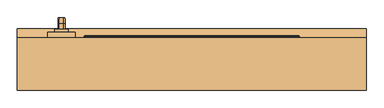
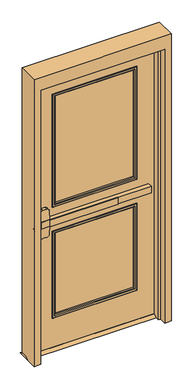
"""IFC4 building model written with IfcOpenShell, lengths in millimetres: door geometry, Дверь-Наружная-Одинарная-Две_Свет : Дверь-Наружная-Одинарная-Две_Свет."""

from ifc_helpers import new_model, si_unit, point, frame, frame_2d, origin, place, context, project, spatial, polyline, circle_curve, ellipse_curve, trimmed, segment, composite_curve, outline, extrude, faceted_brep, source, transform, mapped, element, save
from ifc_brep_helpers import plane_surface, cylinder_surface, revolved_surface, advanced_brep


def door_4063ef7d(model_context):
    return source(origin(), model_context, "Body", "SolidModel", [
        extrude(outline(polyline([(36.35, 15.0), (81.35, 15.0), (106.75, 0.0), (10.95, 0.0), (36.35, 15.0)])), frame((-500.0, 0.0, 0.0), z_axis=(1.0, 0.0, 0.0), x_axis=(0.0, 1.0, 0.0)), (0.0, 0.0, 1.0), 1000.0),
        extrude(outline(polyline([(148.95, -1.75), (-342.05, -1.75), (-342.05, 4.6), (148.95, 4.6), (148.95, -1.75)])), frame((0.0, 0.0, 974.6), z_axis=(0.0, 0.0, 1.0), x_axis=(1.0, 0.0, 0.0)), (0.0, 0.0, 1.0), 50.8),
        advanced_brep(
        [(-405.55, 4.6, 1025.4), (-405.55, 4.6, 974.6), (-342.05, 4.6, 974.6), (394.45, 4.6, 974.6), (394.45, 4.6, 1025.4), (-342.05, 4.6, 1025.4), (394.45, 36.35, 1025.4), (394.45, 36.35, 974.6), (-342.05, 36.35, 974.6), (-342.05, 36.35, 911.1), (-361.1, 36.35, 892.05), (-386.5, 36.35, 892.05), (-405.55, 36.35, 911.1), (-405.55, 36.35, 1088.9), (-386.5, 36.35, 1107.95), (-361.1, 36.35, 1107.95), (-342.05, 36.35, 1088.9), (-342.05, 36.35, 1025.4), (-342.05, 7.7752467, 1025.4), (-405.55, 7.7752467, 1025.4), (-405.55, 12.7854269, 1088.9), (-405.55, 12.7854269, 911.1), (-405.55, 7.7752467, 974.6), (-342.05, 7.7752467, 974.6), (-342.05, 12.7854269, 911.1), (-342.05, 12.7854269, 1088.9), (-386.5, 14.288481, 1107.95), (-361.1, 14.288481, 1107.95), (-361.1, 14.288481, 892.05), (-386.5, 14.288481, 892.05)],
        [
            (0, 1),
            (1, 2),
            (2, 3),
            (3, 4),
            (4, 5),
            (5, 0),
            (6, 7),
            (7, 8),
            (8, 9),
            (9, 10, circle_curve(frame((-361.1, 36.35, 911.1), z_axis=(0.0, 1.0, 0.0), x_axis=(1.0, 0.0, 0.0)), 19.05)),
            (10, 11),
            (11, 12, circle_curve(frame((-386.5, 36.35, 911.1), z_axis=(0.0, 1.0, 0.0), x_axis=(1.0, 0.0, 0.0)), 19.05)),
            (12, 13),
            (13, 14, circle_curve(frame((-386.5, 36.35, 1088.9), z_axis=(0.0, 1.0, 0.0), x_axis=(1.0, 0.0, 0.0)), 19.05)),
            (14, 15),
            (15, 16, circle_curve(frame((-361.1, 36.35, 1088.9), z_axis=(0.0, 1.0, 0.0), x_axis=(1.0, 0.0, 0.0)), 19.05)),
            (16, 17),
            (17, 6),
            (4, 6),
            (17, 18),
            (18, 19),
            (19, 0),
            (19, 20),
            (20, 13),
            (12, 21),
            (21, 22),
            (22, 1),
            (7, 3),
            (22, 23),
            (23, 8),
            (23, 24),
            (24, 9),
            (16, 25),
            (25, 18),
            (14, 26),
            (26, 27),
            (27, 15),
            (10, 28),
            (28, 29),
            (29, 11),
            (24, 28, ellipse_curve(frame((-361.1, 12.7854269, 911.1), z_axis=(0.0, 0.9969018152893365, 0.07865602756830282), x_axis=(0.0, -0.07865602756830208, 0.9969018152893365)), 19.1092038, 19.05)),
            (27, 25, ellipse_curve(frame((-361.1, 12.7854269, 1088.9), z_axis=(0.0, 0.9969018152893376, -0.07865602756828934), x_axis=(0.0, -0.078656027568288, -0.9969018152893377)), 19.1092038, 19.05)),
            (20, 26, ellipse_curve(frame((-386.5, 12.7854269, 1088.9), z_axis=(0.0, 0.9969018152893376, -0.07865602756828934), x_axis=(0.0, -0.078656027568288, -0.9969018152893377)), 19.1092038, 19.05)),
            (29, 21, ellipse_curve(frame((-386.5, 12.7854269, 911.1), z_axis=(0.0, 0.9969018152893365, 0.07865602756830282), x_axis=(0.0, -0.07865602756830208, 0.9969018152893365)), 19.1092038, 19.05)),
        ],
        [
            plane_surface(frame((-405.55, 4.6, 1025.4), z_axis=(0.0, -1.0, 0.0), x_axis=(-1.0, 0.0, 0.0))),
            plane_surface(frame((-405.55, 36.35, 1025.4), z_axis=(0.0, 1.0, 0.0), x_axis=(1.0, 0.0, 0.0))),
            plane_surface(frame((394.45, 4.6, 1025.4), z_axis=(0.0, 0.0, 1.0), x_axis=(0.0, 1.0, 0.0))),
            plane_surface(frame((-405.55, 4.6, 1025.4), z_axis=(-1.0, 0.0, 0.0), x_axis=(0.0, 1.0, 0.0))),
            plane_surface(frame((-405.55, 4.6, 974.6), z_axis=(0.0, 0.0, -1.0), x_axis=(0.0, 1.0, 0.0))),
            plane_surface(frame((394.45, 4.6, 974.6), z_axis=(1.0, 0.0, 0.0), x_axis=(0.0, 1.0, 0.0))),
            plane_surface(frame((-342.05, 7.7752467, 911.1), z_axis=(1.0, 0.0, 0.0), x_axis=(0.0, 1.0, 0.0))),
            plane_surface(frame((-361.1, 7.7752467, 1107.95), z_axis=(0.0, 0.0, 1.0), x_axis=(0.0, 1.0, 0.0))),
            plane_surface(frame((-386.5, 7.7752467, 892.05), z_axis=(0.0, 0.0, -1.0), x_axis=(0.0, 1.0, 0.0))),
            cylinder_surface(frame((-361.1, 36.35, 911.1), z_axis=(0.0, -1.0, 0.0), x_axis=(1.0, 0.0, 0.0)), 19.05),
            cylinder_surface(frame((-361.1, 36.35, 1088.9), z_axis=(0.0, -1.0, 0.0), x_axis=(1.0, 0.0, 0.0)), 19.05),
            cylinder_surface(frame((-386.5, 36.35, 1088.9), z_axis=(0.0, -1.0, 0.0), x_axis=(1.0, 0.0, 0.0)), 19.05),
            cylinder_surface(frame((-386.5, 36.35, 911.1), z_axis=(0.0, -1.0, 0.0), x_axis=(1.0, 0.0, 0.0)), 19.05),
            plane_surface(frame((-342.05, 7.7752467, 1025.4), z_axis=(0.0, -0.9969018152893376, 0.07865602756828934), x_axis=(-1.0, 0.0, 0.0))),
            plane_surface(frame((-342.05, 14.288481, 892.05), z_axis=(0.0, -0.9969018152893365, -0.07865602756830282), x_axis=(-1.0, 0.0, 0.0))),
        ],
        [
            (0, [[1, 2, 3, 4, 5, 6]]),
            (1, [[7, 8, 9, 10, 11, 12, 13, 14, 15, 16, 17, 18]]),
            (2, [[19, -18, 20, 21, 22, -6, -5]]),
            (3, [[-1, -22, 23, 24, -13, 25, 26, 27]]),
            (4, [[28, -3, -2, -27, 29, 30, -8]]),
            (5, [[-4, -28, -7, -19]]),
            (6, [[-9, -30, 31, 32]]),
            (6, [[-17, 33, 34, -20]]),
            (7, [[-15, 35, 36, 37]]),
            (8, [[-11, 38, 39, 40]]),
            (9, [[-10, -32, 41, -38]]),
            (10, [[-16, -37, 42, -33]]),
            (11, [[-14, -24, 43, -35]]),
            (12, [[-12, -40, 44, -25]]),
            (13, [[-21, -34, -42, -36, -43, -23]]),
            (14, [[-26, -44, -39, -41, -31, -29]]),
        ],
    ),
        advanced_brep(
        [(-383.8, 96.35, 1001.190625), (-383.8, 96.35, 998.809375), (-380.228125, 96.35, 995.2375), (-367.3715406, 96.35, 995.2375), (-363.8, 96.35, 998.8090406), (-363.8, 96.35, 1001.190625), (-367.371875, 96.35, 1004.7625), (-380.228125, 96.35, 1004.7625), (-383.8, 96.35, 874.609375), (-380.228125, 96.35, 871.0375), (-367.371875, 96.35, 871.0375), (-363.8, 96.35, 874.609375), (-363.8, 96.35, 876.9909594), (-367.3715406, 96.35, 880.5625), (-380.228125, 96.35, 880.5625), (-383.8, 96.35, 876.990625), (-383.8, 121.75, 1001.190625), (-383.8, 135.640625, 987.3), (-383.8, 135.640625, 888.5), (-383.8, 121.75, 874.609375), (-383.8, 121.75, 876.990625), (-383.8, 133.259375, 888.5), (-383.8, 133.259375, 987.3), (-383.8, 121.75, 998.809375), (-380.228125, 121.75, 995.2375), (-367.3715406, 121.75, 995.2375), (-363.8, 121.75, 998.8090406), (-363.8, 133.2590406, 987.3), (-363.8, 133.2590406, 888.5), (-363.8, 121.75, 876.9909594), (-363.8, 121.75, 874.609375), (-363.8, 135.640625, 888.5), (-363.8, 135.640625, 987.3), (-363.8, 121.75, 1001.190625), (-367.371875, 121.75, 1004.7625), (-380.228125, 121.75, 1004.7625), (-380.228125, 129.6875, 987.3), (-367.3715406, 129.6875, 987.3), (-367.371875, 139.2125, 987.3), (-380.228125, 139.2125, 987.3), (-380.228125, 129.6875, 888.5), (-367.3715406, 129.6875, 888.5), (-367.371875, 139.2125, 888.5), (-380.228125, 139.2125, 888.5), (-380.228125, 121.75, 880.5625), (-367.3715406, 121.75, 880.5625), (-367.371875, 121.75, 871.0375), (-380.228125, 121.75, 871.0375)],
        [
            (0, 1),
            (1, 2, circle_curve(frame((-380.228125, 96.35, 998.809375), z_axis=(0.0, -1.0, 0.0), x_axis=(0.0, 0.0, 1.0)), 3.571875)),
            (2, 3),
            (3, 4, circle_curve(frame((-367.3715406, 96.35, 998.8090406), z_axis=(0.0, -1.0, 0.0), x_axis=(0.0, 0.0, 1.0)), 3.5715406)),
            (4, 5),
            (5, 6, circle_curve(frame((-367.371875, 96.35, 1001.190625), z_axis=(0.0, -1.0, 0.0), x_axis=(0.0, 0.0, 1.0)), 3.571875)),
            (6, 7),
            (7, 0, circle_curve(frame((-380.228125, 96.35, 1001.190625), z_axis=(0.0, -1.0, 0.0), x_axis=(0.0, 0.0, 1.0)), 3.571875)),
            (8, 9, circle_curve(frame((-380.228125, 96.35, 874.609375), z_axis=(0.0, -1.0, 0.0), x_axis=(0.0, 0.0, -1.0)), 3.571875)),
            (9, 10),
            (10, 11, circle_curve(frame((-367.371875, 96.35, 874.609375), z_axis=(0.0, -1.0, 0.0), x_axis=(0.0, 0.0, -1.0)), 3.571875)),
            (11, 12),
            (12, 13, circle_curve(frame((-367.3715406, 96.35, 876.9909594), z_axis=(0.0, -1.0, 0.0), x_axis=(0.0, 0.0, -1.0)), 3.5715406)),
            (13, 14),
            (14, 15, circle_curve(frame((-380.228125, 96.35, 876.990625), z_axis=(0.0, -1.0, 0.0), x_axis=(0.0, 0.0, -1.0)), 3.571875)),
            (15, 8),
            (0, 16),
            (16, 17, circle_curve(frame((-383.8, 121.75, 987.3), z_axis=(-1.0, 0.0, 0.0), x_axis=(0.0, 0.0, 1.0)), 13.890625)),
            (17, 18),
            (18, 19, circle_curve(frame((-383.8, 121.75, 888.5), z_axis=(-1.0, 0.0, 0.0), x_axis=(0.0, 1.0, 0.0)), 13.890625)),
            (19, 8),
            (15, 20),
            (20, 21, circle_curve(frame((-383.8, 121.75, 888.5), z_axis=(1.0, 0.0, 0.0), x_axis=(0.0, 1.0, 0.0)), 11.509375)),
            (21, 22),
            (22, 23, circle_curve(frame((-383.8, 121.75, 987.3), z_axis=(1.0, 0.0, 0.0), x_axis=(0.0, 0.0, 1.0)), 11.509375)),
            (23, 1),
            (23, 24, circle_curve(frame((-380.228125, 121.75, 998.809375), z_axis=(0.0, -1.0, 0.0), x_axis=(0.0, 0.0, 1.0)), 3.571875)),
            (24, 2),
            (24, 25),
            (25, 3),
            (25, 26, circle_curve(frame((-367.3715406, 121.75, 998.8090406), z_axis=(0.0, -1.0, 0.0), x_axis=(0.0, 0.0, 1.0)), 3.5715406)),
            (26, 4),
            (26, 27, circle_curve(frame((-363.8, 121.75, 987.3), z_axis=(-1.0, 0.0, 0.0), x_axis=(0.0, 0.0, 1.0)), 11.5090406)),
            (27, 28),
            (28, 29, circle_curve(frame((-363.8, 121.75, 888.5), z_axis=(-1.0, 0.0, 0.0), x_axis=(0.0, 1.0, 0.0)), 11.5090406)),
            (29, 12),
            (11, 30),
            (30, 31, circle_curve(frame((-363.8, 121.75, 888.5), z_axis=(1.0, 0.0, 0.0), x_axis=(0.0, 1.0, 0.0)), 13.890625)),
            (31, 32),
            (32, 33, circle_curve(frame((-363.8, 121.75, 987.3), z_axis=(1.0, 0.0, 0.0), x_axis=(0.0, 0.0, 1.0)), 13.890625)),
            (33, 5),
            (33, 34, circle_curve(frame((-367.371875, 121.75, 1001.190625), z_axis=(0.0, -1.0, 0.0), x_axis=(0.0, 0.0, 1.0)), 3.571875)),
            (34, 6),
            (34, 35),
            (35, 7),
            (35, 16, circle_curve(frame((-380.228125, 121.75, 1001.190625), z_axis=(0.0, -1.0, 0.0), x_axis=(0.0, 0.0, 1.0)), 3.571875)),
            (36, 24, circle_curve(frame((-380.228125, 121.75, 987.3), z_axis=(1.0, 0.0, 0.0), x_axis=(0.0, 0.0, 1.0)), 7.9375)),
            (22, 36, circle_curve(frame((-380.228125, 133.259375, 987.3), z_axis=(0.0, 0.0, 1.0), x_axis=(0.0, 1.0, 0.0)), 3.571875)),
            (37, 25, circle_curve(frame((-367.3715406, 121.75, 987.3), z_axis=(1.0, 0.0, 0.0), x_axis=(0.0, 0.0, 1.0)), 7.9375)),
            (36, 37),
            (37, 27, circle_curve(frame((-367.3715406, 133.2590406, 987.3), z_axis=(0.0, 0.0, 1.0), x_axis=(0.0, 1.0, 0.0)), 3.5715406)),
            (38, 34, circle_curve(frame((-367.371875, 121.75, 987.3), z_axis=(1.0, 0.0, 0.0), x_axis=(0.0, 0.0, 1.0)), 17.4625)),
            (32, 38, circle_curve(frame((-367.371875, 135.640625, 987.3), z_axis=(0.0, 0.0, 1.0), x_axis=(0.0, 1.0, 0.0)), 3.571875)),
            (39, 35, circle_curve(frame((-380.228125, 121.75, 987.3), z_axis=(1.0, 0.0, 0.0), x_axis=(0.0, 0.0, 1.0)), 17.4625)),
            (38, 39),
            (39, 17, circle_curve(frame((-380.228125, 135.640625, 987.3), z_axis=(0.0, 0.0, 1.0), x_axis=(0.0, 1.0, 0.0)), 3.571875)),
            (21, 40, circle_curve(frame((-380.228125, 133.259375, 888.5), z_axis=(0.0, 0.0, 1.0), x_axis=(0.0, 1.0, 0.0)), 3.571875)),
            (40, 36),
            (40, 41),
            (41, 37),
            (41, 28, circle_curve(frame((-367.3715406, 133.2590406, 888.5), z_axis=(0.0, 0.0, 1.0), x_axis=(0.0, 1.0, 0.0)), 3.5715406)),
            (31, 42, circle_curve(frame((-367.371875, 135.640625, 888.5), z_axis=(0.0, 0.0, 1.0), x_axis=(0.0, 1.0, 0.0)), 3.571875)),
            (42, 38),
            (42, 43),
            (43, 39),
            (43, 18, circle_curve(frame((-380.228125, 135.640625, 888.5), z_axis=(0.0, 0.0, 1.0), x_axis=(0.0, 1.0, 0.0)), 3.571875)),
            (44, 40, circle_curve(frame((-380.228125, 121.75, 888.5), z_axis=(1.0, 0.0, 0.0), x_axis=(0.0, 1.0, 0.0)), 7.9375)),
            (20, 44, circle_curve(frame((-380.228125, 121.75, 876.990625), z_axis=(0.0, 1.0, 0.0), x_axis=(0.0, 0.0, -1.0)), 3.571875)),
            (45, 41, circle_curve(frame((-367.3715406, 121.75, 888.5), z_axis=(1.0, 0.0, 0.0), x_axis=(0.0, 1.0, 0.0)), 7.9375)),
            (44, 45),
            (45, 29, circle_curve(frame((-367.3715406, 121.75, 876.9909594), z_axis=(0.0, 1.0, 0.0), x_axis=(0.0, 0.0, -1.0)), 3.5715406)),
            (46, 42, circle_curve(frame((-367.371875, 121.75, 888.5), z_axis=(1.0, 0.0, 0.0), x_axis=(0.0, 1.0, 0.0)), 17.4625)),
            (30, 46, circle_curve(frame((-367.371875, 121.75, 874.609375), z_axis=(0.0, 1.0, 0.0), x_axis=(0.0, 0.0, -1.0)), 3.571875)),
            (47, 43, circle_curve(frame((-380.228125, 121.75, 888.5), z_axis=(1.0, 0.0, 0.0), x_axis=(0.0, 1.0, 0.0)), 17.4625)),
            (46, 47),
            (47, 19, circle_curve(frame((-380.228125, 121.75, 874.609375), z_axis=(0.0, 1.0, 0.0), x_axis=(0.0, 0.0, -1.0)), 3.571875)),
            (14, 44),
            (13, 45),
            (10, 46),
            (9, 47),
        ],
        [
            plane_surface(frame((-373.8, 96.35, 1000.0), z_axis=(0.0, -1.0, 0.0), x_axis=(1.0, 0.0, 0.0))),
            plane_surface(frame((-373.8, 96.35, 875.8), z_axis=(0.0, -1.0, 0.0), x_axis=(1.0, 0.0, 0.0))),
            plane_surface(frame((-383.8, 96.35, 1001.190625), z_axis=(-1.0, 0.0, 0.0), x_axis=(0.0, 1.0, 0.0))),
            cylinder_surface(frame((-380.228125, 96.35, 998.809375), z_axis=(0.0, -1.0, 0.0), x_axis=(0.0, 0.0, 1.0)), 3.571875),
            plane_surface(frame((-380.228125, 96.35, 995.2375), z_axis=(0.0, 0.0, -1.0), x_axis=(0.0, 1.0, 0.0))),
            cylinder_surface(frame((-367.3715406, 96.35, 998.8090406), z_axis=(0.0, -1.0, 0.0), x_axis=(0.0, 0.0, 1.0)), 3.5715406),
            plane_surface(frame((-363.8, 96.35, 998.8090406), z_axis=(1.0, 0.0, 0.0), x_axis=(0.0, 1.0, 0.0))),
            cylinder_surface(frame((-367.371875, 96.35, 1001.190625), z_axis=(0.0, -1.0, 0.0), x_axis=(0.0, 0.0, 1.0)), 3.571875),
            plane_surface(frame((-367.371875, 96.35, 1004.7625), z_axis=(0.0, 0.0, 1.0), x_axis=(0.0, 1.0, 0.0))),
            cylinder_surface(frame((-380.228125, 96.35, 1001.190625), z_axis=(0.0, -1.0, 0.0), x_axis=(0.0, 0.0, 1.0)), 3.571875),
            revolved_surface(trimmed(ellipse_curve(frame((-380.228125, 121.75, 998.809375), z_axis=(0.0, -1.0, 0.0), x_axis=(0.0, 0.0, 1.0)), 3.571875, 3.571875), [point((-383.8, 121.75, 998.809375))], [point((-380.228125, 121.75, 995.2375))], True, "CARTESIAN"), (-373.8, 121.75, 987.3), (-1.0, 0.0, 0.0)),
            revolved_surface(polyline([(-380.228125, 121.75, 995.2375), (-367.3715406, 121.75, 995.2375)]), (-373.8, 121.75, 987.3), (-1.0, 0.0, 0.0)),
            revolved_surface(trimmed(ellipse_curve(frame((-367.3715406, 121.75, 998.8090406), z_axis=(0.0, -1.0, 0.0), x_axis=(0.0, 0.0, 1.0)), 3.5715406, 3.5715406), [point((-367.3715406, 121.75, 995.2375))], [point((-363.8, 121.75, 998.8090406))], True, "CARTESIAN"), (-373.8, 121.75, 987.3), (-1.0, 0.0, 0.0)),
            revolved_surface(trimmed(ellipse_curve(frame((-367.371875, 121.75, 1001.190625), z_axis=(0.0, -1.0, 0.0), x_axis=(0.0, 0.0, 1.0)), 3.571875, 3.571875), [point((-363.8, 121.75, 1001.190625))], [point((-367.371875, 121.75, 1004.7625))], True, "CARTESIAN"), (-373.8, 121.75, 987.3), (-1.0, 0.0, 0.0)),
            cylinder_surface(frame((-373.8, 121.75, 987.3), z_axis=(-1.0, 0.0, 0.0), x_axis=(0.0, 0.0, 1.0)), 17.4625),
            revolved_surface(trimmed(ellipse_curve(frame((-380.228125, 121.75, 1001.190625), z_axis=(0.0, -1.0, 0.0), x_axis=(0.0, 0.0, 1.0)), 3.571875, 3.571875), [point((-380.228125, 121.75, 1004.7625))], [point((-383.8, 121.75, 1001.190625))], True, "CARTESIAN"), (-373.8, 121.75, 987.3), (-1.0, 0.0, 0.0)),
            cylinder_surface(frame((-380.228125, 133.259375, 987.3), z_axis=(0.0, 0.0, 1.0), x_axis=(0.0, 1.0, 0.0)), 3.571875),
            plane_surface(frame((-380.228125, 129.6875, 987.3), z_axis=(0.0, -1.0, 0.0), x_axis=(0.0, 0.0, -1.0))),
            cylinder_surface(frame((-367.3715406, 133.2590406, 987.3), z_axis=(0.0, 0.0, 1.0), x_axis=(0.0, 1.0, 0.0)), 3.5715406),
            cylinder_surface(frame((-367.371875, 135.640625, 987.3), z_axis=(0.0, 0.0, 1.0), x_axis=(0.0, 1.0, 0.0)), 3.571875),
            plane_surface(frame((-367.371875, 139.2125, 987.3), z_axis=(0.0, 1.0, 0.0), x_axis=(0.0, 0.0, -1.0))),
            cylinder_surface(frame((-380.228125, 135.640625, 987.3), z_axis=(0.0, 0.0, 1.0), x_axis=(0.0, 1.0, 0.0)), 3.571875),
            revolved_surface(trimmed(ellipse_curve(frame((-380.228125, 133.259375, 888.5), z_axis=(0.0, 0.0, 1.0), x_axis=(0.0, 1.0, 0.0)), 3.571875, 3.571875), [point((-383.8, 133.259375, 888.5))], [point((-380.228125, 129.6875, 888.5))], True, "CARTESIAN"), (-373.8, 121.75, 888.5), (-1.0, 0.0, 0.0)),
            revolved_surface(polyline([(-380.228125, 129.6875, 888.5), (-367.3715406, 129.6875, 888.5)]), (-373.8, 121.75, 888.5), (-1.0, 0.0, 0.0)),
            revolved_surface(trimmed(ellipse_curve(frame((-367.3715406, 133.2590406, 888.5), z_axis=(0.0, 0.0, 1.0), x_axis=(0.0, 1.0, 0.0)), 3.5715406, 3.5715406), [point((-367.3715406, 129.6875, 888.5))], [point((-363.8, 133.2590406, 888.5))], True, "CARTESIAN"), (-373.8, 121.75, 888.5), (-1.0, 0.0, 0.0)),
            revolved_surface(trimmed(ellipse_curve(frame((-367.371875, 135.640625, 888.5), z_axis=(0.0, 0.0, 1.0), x_axis=(0.0, 1.0, 0.0)), 3.571875, 3.571875), [point((-363.8, 135.640625, 888.5))], [point((-367.371875, 139.2125, 888.5))], True, "CARTESIAN"), (-373.8, 121.75, 888.5), (-1.0, 0.0, 0.0)),
            cylinder_surface(frame((-373.8, 121.75, 888.5), z_axis=(-1.0, 0.0, 0.0), x_axis=(0.0, 1.0, 0.0)), 17.4625),
            revolved_surface(trimmed(ellipse_curve(frame((-380.228125, 135.640625, 888.5), z_axis=(0.0, 0.0, 1.0), x_axis=(0.0, 1.0, 0.0)), 3.571875, 3.571875), [point((-380.228125, 139.2125, 888.5))], [point((-383.8, 135.640625, 888.5))], True, "CARTESIAN"), (-373.8, 121.75, 888.5), (-1.0, 0.0, 0.0)),
            cylinder_surface(frame((-380.228125, 121.75, 876.990625), z_axis=(0.0, 1.0, 0.0), x_axis=(0.0, 0.0, -1.0)), 3.571875),
            plane_surface(frame((-380.228125, 121.75, 880.5625), z_axis=(0.0, 0.0, 1.0), x_axis=(0.0, -1.0, 0.0))),
            cylinder_surface(frame((-367.3715406, 121.75, 876.9909594), z_axis=(0.0, 1.0, 0.0), x_axis=(0.0, 0.0, -1.0)), 3.5715406),
            cylinder_surface(frame((-367.371875, 121.75, 874.609375), z_axis=(0.0, 1.0, 0.0), x_axis=(0.0, 0.0, -1.0)), 3.571875),
            plane_surface(frame((-367.371875, 121.75, 871.0375), z_axis=(0.0, 0.0, -1.0), x_axis=(0.0, -1.0, 0.0))),
            cylinder_surface(frame((-380.228125, 121.75, 874.609375), z_axis=(0.0, 1.0, 0.0), x_axis=(0.0, 0.0, -1.0)), 3.571875),
        ],
        [
            (0, [[1, 2, 3, 4, 5, 6, 7, 8]]),
            (1, [[9, 10, 11, 12, 13, 14, 15, 16]]),
            (2, [[-1, 17, 18, 19, 20, 21, -16, 22, 23, 24, 25, 26]]),
            (3, [[-2, -26, 27, 28]]),
            (4, [[-3, -28, 29, 30]]),
            (5, [[-4, -30, 31, 32]]),
            (6, [[-5, -32, 33, 34, 35, 36, -12, 37, 38, 39, 40, 41]]),
            (7, [[-6, -41, 42, 43]]),
            (8, [[-7, -43, 44, 45]]),
            (9, [[-8, -45, 46, -17]]),
            (10, [[47, -27, -25, 48]]),
            (11, [[49, -29, -47, 50]]),
            (12, [[-33, -31, -49, 51]]),
            (13, [[52, -42, -40, 53]]),
            (14, [[54, -44, -52, 55]]),
            (15, [[-18, -46, -54, 56]]),
            (16, [[-48, -24, 57, 58]]),
            (17, [[-50, -58, 59, 60]]),
            (18, [[-51, -60, 61, -34]]),
            (19, [[-53, -39, 62, 63]]),
            (20, [[-55, -63, 64, 65]]),
            (21, [[-56, -65, 66, -19]]),
            (22, [[67, -57, -23, 68]]),
            (23, [[69, -59, -67, 70]]),
            (24, [[-35, -61, -69, 71]]),
            (25, [[72, -62, -38, 73]]),
            (26, [[74, -64, -72, 75]]),
            (27, [[-20, -66, -74, 76]]),
            (28, [[-68, -22, -15, 77]]),
            (29, [[-70, -77, -14, 78]]),
            (30, [[-71, -78, -13, -36]]),
            (31, [[-73, -37, -11, 79]]),
            (32, [[-75, -79, -10, 80]]),
            (33, [[-76, -80, -9, -21]]),
        ],
    ),
        extrude(outline(composite_curve([segment(trimmed(circle_curve(frame_2d((1098.8, -373.8)), 19.0), [point((1098.8, -392.8))], [point((1098.8, -354.8))], False, "CARTESIAN"), True, "CONTINUOUS"), segment(trimmed(circle_curve(frame_2d((1098.8, -373.8)), 19.0), [point((1098.8, -354.8))], [point((1098.8, -392.8))], False, "CARTESIAN"), True, "CONTINUOUS")], self_intersect=False)), frame((0.0, 96.35, 0.0), z_axis=(0.0, 1.0, 0.0), x_axis=(0.0, 0.0, 1.0)), (0.0, 0.0, 1.0), 8.73125),
        extrude(outline(composite_curve([segment(trimmed(circle_curve(frame_2d((1094.2338574, -373.8)), 90.1286291), [point((1175.0, -333.8))], [point((1175.0, -413.8))], False, "CARTESIAN"), True, "CONTINUOUS"), segment(polyline([(1175.0, -413.8), (825.0, -413.8)]), True, "CONTINUOUS"), segment(trimmed(circle_curve(frame_2d((905.7661426, -373.8)), 90.1286291), [point((825.0, -413.8))], [point((825.0, -333.8))], False, "CARTESIAN"), True, "CONTINUOUS"), segment(polyline([(825.0, -333.8), (1175.0, -333.8)]), True, "CONTINUOUS")], self_intersect=False)), frame((0.0, 81.35, 0.0), z_axis=(0.0, 1.0, 0.0), x_axis=(0.0, 0.0, 1.0)), (0.0, 0.0, 1.0), 15.0),
        extrude(outline(polyline([(2100.0, -450.0), (15.0, -450.0), (15.0, 450.0), (2100.0, 450.0), (2100.0, -450.0)]), holes=[polyline([(1950.0, -300.0), (1950.0, 300.0), (1100.0, 300.0), (1100.0, -300.0), (1950.0, -300.0)]), polyline([(900.0, -300.0), (900.0, 300.0), (250.0, 300.0), (250.0, -300.0), (900.0, -300.0)])]), frame((0.0, 36.35, 0.0), z_axis=(0.0, 1.0, 0.0), x_axis=(0.0, 0.0, 1.0)), (0.0, 0.0, 1.0), 45.0),
        faceted_brep([(450.0, 31.5875, 0.0), (450.0, 81.35, 0.0), (500.0, 81.35, 0.0), (500.0, -68.65, 0.0), (450.0, -68.65, 0.0), (450.0, -19.4375, 0.0), (434.125, -19.4375, 0.0), (434.125, 31.5875, 0.0), (450.0, 31.5875, 2100.0), (450.0, 81.35, 2100.0), (-450.0, 81.35, 2100.0), (-450.0, 81.35, 0.0), (-500.0, 81.35, 0.0), (-500.0, 81.35, 2200.0), (500.0, 81.35, 2200.0), (500.0, -68.65, 2200.0), (-500.0, -68.65, 2200.0), (-500.0, -68.65, 0.0), (-450.0, -68.65, 0.0), (-450.0, -68.65, 2100.0), (450.0, -68.65, 2100.0), (450.0, -19.4375, 2100.0), (-450.0, -19.4375, 2100.0), (-450.0, -19.4375, 0.0), (-434.125, -19.4375, 0.0), (-434.125, -19.4375, 2084.125), (434.125, -19.4375, 2084.125), (434.125, 31.5875, 2084.125), (-434.125, 31.5875, 2084.125), (-434.125, 31.5875, 0.0), (-450.0, 31.5875, 0.0), (-450.0, 31.5875, 2100.0)], [[[0, 1, 2, 3, 4, 5, 6, 7]], [[1, 0, 8, 9]], [[2, 1, 9, 10, 11, 12, 13, 14]], [[3, 2, 14, 15]], [[4, 3, 15, 16, 17, 18, 19, 20]], [[5, 4, 20, 21]], [[6, 5, 21, 22, 23, 24, 25, 26]], [[7, 6, 26, 27]], [[0, 7, 27, 28, 29, 30, 31, 8]], [[9, 8, 31, 10]], [[20, 19, 22, 21]], [[26, 25, 28, 27]], [[12, 11, 30, 29, 24, 23, 18, 17]], [[11, 10, 31, 30]], [[13, 12, 17, 16]], [[19, 18, 23, 22]], [[25, 24, 29, 28]], [[15, 14, 13, 16]]]),
        extrude(outline(polyline([(300.0, 48.85), (-300.0, 48.85), (-300.0, 68.85), (300.0, 68.85), (300.0, 48.85)])), frame((0.0, 0.0, 1100.0), z_axis=(0.0, 0.0, 1.0), x_axis=(1.0, 0.0, 0.0)), (0.0, 0.0, 1.0), 850.0),
        extrude(outline(polyline([(300.0, 48.85), (-300.0, 48.85), (-300.0, 68.85), (300.0, 68.85), (300.0, 48.85)])), frame((0.0, 0.0, 250.0), z_axis=(0.0, 0.0, 1.0), x_axis=(1.0, 0.0, 0.0)), (0.0, 0.0, 1.0), 650.0),
        advanced_brep(
        [(-300.0, 68.85, 1950.0), (-300.0, 81.35, 1950.0), (-300.0, 81.35, 1100.0), (-300.0, 68.85, 1100.0), (-288.0, 82.35, 1938.0), (-288.0, 68.85, 1938.0), (-288.0, 68.85, 1112.0), (-288.0, 82.35, 1112.0), (-293.0, 87.35, 1943.0), (-293.0, 87.35, 1107.0), (-308.0, 85.35, 1958.0), (-306.0, 87.35, 1956.0), (-306.0, 87.35, 1094.0), (-308.0, 85.35, 1092.0), (-308.0, 81.35, 1958.0), (-308.0, 81.35, 1092.0), (300.0, 81.35, 1100.0), (300.0, 68.85, 1100.0), (288.0, 68.85, 1112.0), (288.0, 82.35, 1112.0), (293.0, 87.35, 1107.0), (306.0, 87.35, 1094.0), (308.0, 85.35, 1092.0), (308.0, 81.35, 1092.0), (300.0, 81.35, 1950.0), (300.0, 68.85, 1950.0), (288.0, 68.85, 1938.0), (288.0, 82.35, 1938.0), (293.0, 87.35, 1943.0), (306.0, 87.35, 1956.0), (308.0, 85.35, 1958.0), (308.0, 81.35, 1958.0)],
        [
            (0, 1),
            (1, 2),
            (2, 3),
            (3, 0),
            (4, 5),
            (5, 6),
            (6, 7),
            (7, 4),
            (8, 4, ellipse_curve(frame((-293.0, 82.35, 1943.0), z_axis=(-0.7071067811865475, 0.0, -0.7071067811865475), x_axis=(-0.7071067811865474, 0.0, 0.7071067811865476)), 7.0710678, 5.0)),
            (7, 9, ellipse_curve(frame((-293.0, 82.35, 1107.0), z_axis=(-0.7071067811865475, 0.0, 0.7071067811865475), x_axis=(0.7071067811865474, 0.0, 0.7071067811865476)), 7.0710678, 5.0)),
            (9, 8),
            (10, 11, ellipse_curve(frame((-306.0, 85.35, 1956.0), z_axis=(-0.7071067811865475, 0.0, -0.7071067811865475), x_axis=(-0.7071067811865474, 0.0, 0.7071067811865476)), 2.8284271, 2.0)),
            (11, 12),
            (12, 13, ellipse_curve(frame((-306.0, 85.35, 1094.0), z_axis=(-0.7071067811865475, 0.0, 0.7071067811865475), x_axis=(0.7071067811865474, 0.0, 0.7071067811865476)), 2.8284271, 2.0)),
            (13, 10),
            (14, 10),
            (13, 15),
            (15, 14),
            (2, 16),
            (16, 17),
            (17, 3),
            (6, 18),
            (18, 19),
            (19, 7),
            (19, 20, ellipse_curve(frame((293.0, 82.35, 1107.0), z_axis=(-0.7071067811865475, 0.0, -0.7071067811865475), x_axis=(-0.7071067811865476, 0.0, 0.7071067811865474)), 7.0710678, 5.0)),
            (20, 9),
            (12, 21),
            (21, 22, ellipse_curve(frame((306.0, 85.35, 1094.0), z_axis=(-0.7071067811865475, 0.0, -0.7071067811865475), x_axis=(-0.7071067811865476, 0.0, 0.7071067811865474)), 2.8284271, 2.0)),
            (22, 13),
            (22, 23),
            (23, 15),
            (16, 24),
            (24, 25),
            (25, 17),
            (18, 26),
            (26, 27),
            (27, 19),
            (27, 28, ellipse_curve(frame((293.0, 82.35, 1943.0), z_axis=(0.7071067811865475, 0.0, -0.7071067811865475), x_axis=(-0.7071067811865474, 0.0, -0.7071067811865476)), 7.0710678, 5.0)),
            (28, 20),
            (21, 29),
            (29, 30, ellipse_curve(frame((306.0, 85.35, 1956.0), z_axis=(0.7071067811865475, 0.0, -0.7071067811865475), x_axis=(-0.7071067811865474, 0.0, -0.7071067811865476)), 2.8284271, 2.0)),
            (30, 22),
            (30, 31),
            (31, 23),
            (31, 14),
            (1, 24),
            (0, 25),
            (5, 26),
            (4, 27),
            (8, 28),
            (11, 29),
            (10, 30),
        ],
        [
            plane_surface(frame((-300.0, 81.35, 1950.0), z_axis=(-1.0, 0.0, 0.0), x_axis=(0.0, 0.0, -1.0))),
            plane_surface(frame((-288.0, 68.85, 1938.0), z_axis=(1.0, 0.0, 0.0), x_axis=(0.0, 0.0, -1.0))),
            cylinder_surface(frame((-293.0, 82.35, 1950.0), z_axis=(0.0, 0.0, 1.0), x_axis=(-1.0, 0.0, 0.0)), 5.0),
            cylinder_surface(frame((-306.0, 85.35, 1950.0), z_axis=(0.0, 0.0, 1.0), x_axis=(-1.0, 0.0, 0.0)), 2.0),
            plane_surface(frame((-308.0, 85.35, 1958.0), z_axis=(-1.0, 0.0, 0.0), x_axis=(0.0, 0.0, -1.0))),
            plane_surface(frame((-300.0, 81.35, 1100.0), z_axis=(0.0, 0.0, -1.0), x_axis=(1.0, 0.0, 0.0))),
            plane_surface(frame((-288.0, 68.85, 1112.0), z_axis=(0.0, 0.0, 1.0), x_axis=(1.0, 0.0, 0.0))),
            cylinder_surface(frame((-300.0, 82.35, 1107.0), z_axis=(-1.0, 0.0, 0.0), x_axis=(0.0, 0.0, -1.0)), 5.0),
            cylinder_surface(frame((-300.0, 85.35, 1094.0), z_axis=(-1.0, 0.0, 0.0), x_axis=(0.0, 0.0, -1.0)), 2.0),
            plane_surface(frame((-308.0, 85.35, 1092.0), z_axis=(0.0, 0.0, -1.0), x_axis=(1.0, 0.0, 0.0))),
            plane_surface(frame((300.0, 81.35, 1100.0), z_axis=(1.0, 0.0, 0.0), x_axis=(0.0, 0.0, 1.0))),
            plane_surface(frame((288.0, 68.85, 1112.0), z_axis=(-1.0, 0.0, 0.0), x_axis=(0.0, 0.0, 1.0))),
            cylinder_surface(frame((293.0, 82.35, 1100.0), z_axis=(0.0, 0.0, -1.0), x_axis=(1.0, 0.0, 0.0)), 5.0),
            cylinder_surface(frame((306.0, 85.35, 1100.0), z_axis=(0.0, 0.0, -1.0), x_axis=(1.0, 0.0, 0.0)), 2.0),
            plane_surface(frame((308.0, 85.35, 1092.0), z_axis=(1.0, 0.0, 0.0), x_axis=(0.0, 0.0, 1.0))),
            plane_surface(frame((308.0, 81.35, 1958.0), z_axis=(0.0, -1.0, 0.0), x_axis=(-1.0, 0.0, 0.0))),
            plane_surface(frame((300.0, 81.35, 1950.0), z_axis=(0.0, 0.0, 1.0), x_axis=(-1.0, 0.0, 0.0))),
            plane_surface(frame((300.0, 68.85, 1950.0), z_axis=(0.0, -1.0, 0.0), x_axis=(-1.0, 0.0, 0.0))),
            plane_surface(frame((288.0, 68.85, 1938.0), z_axis=(0.0, 0.0, -1.0), x_axis=(-1.0, 0.0, 0.0))),
            cylinder_surface(frame((300.0, 82.35, 1943.0), z_axis=(1.0, 0.0, 0.0), x_axis=(0.0, 0.0, 1.0)), 5.0),
            plane_surface(frame((293.0, 87.35, 1943.0), z_axis=(0.0, 1.0, 0.0), x_axis=(-1.0, 0.0, 0.0))),
            cylinder_surface(frame((300.0, 85.35, 1956.0), z_axis=(1.0, 0.0, 0.0), x_axis=(0.0, 0.0, 1.0)), 2.0),
            plane_surface(frame((308.0, 85.35, 1958.0), z_axis=(0.0, 0.0, 1.0), x_axis=(-1.0, 0.0, 0.0))),
        ],
        [
            (0, [[1, 2, 3, 4]]),
            (1, [[5, 6, 7, 8]]),
            (2, [[9, -8, 10, 11]]),
            (3, [[12, 13, 14, 15]]),
            (4, [[16, -15, 17, 18]]),
            (5, [[-3, 19, 20, 21]]),
            (6, [[-7, 22, 23, 24]]),
            (7, [[-10, -24, 25, 26]]),
            (8, [[-14, 27, 28, 29]]),
            (9, [[-17, -29, 30, 31]]),
            (10, [[-20, 32, 33, 34]]),
            (11, [[-23, 35, 36, 37]]),
            (12, [[-25, -37, 38, 39]]),
            (13, [[-28, 40, 41, 42]]),
            (14, [[-30, -42, 43, 44]]),
            (15, [[-31, -44, 45, -18], [46, -32, -19, -2]]),
            (16, [[-33, -46, -1, 47]]),
            (17, [[-21, -34, -47, -4], [48, -35, -22, -6]]),
            (18, [[-36, -48, -5, 49]]),
            (19, [[-38, -49, -9, 50]]),
            (20, [[51, -40, -27, -13], [-26, -39, -50, -11]]),
            (21, [[-41, -51, -12, 52]]),
            (22, [[-43, -52, -16, -45]]),
        ],
    ),
        advanced_brep(
        [(-300.0, 48.85, 1100.0), (-300.0, 36.35, 1100.0), (-300.0, 36.35, 1950.0), (-300.0, 48.85, 1950.0), (-288.0, 35.35, 1112.0), (-288.0, 48.85, 1112.0), (-288.0, 48.85, 1938.0), (-288.0, 35.35, 1938.0), (-293.0, 30.35, 1107.0), (-293.0, 30.35, 1943.0), (-308.0, 32.35, 1092.0), (-306.0, 30.35, 1094.0), (-306.0, 30.35, 1956.0), (-308.0, 32.35, 1958.0), (-308.0, 36.35, 1092.0), (-308.0, 36.35, 1958.0), (300.0, 36.35, 1950.0), (300.0, 48.85, 1950.0), (288.0, 48.85, 1938.0), (288.0, 35.35, 1938.0), (293.0, 30.35, 1943.0), (306.0, 30.35, 1956.0), (308.0, 32.35, 1958.0), (308.0, 36.35, 1958.0), (300.0, 36.35, 1100.0), (300.0, 48.85, 1100.0), (288.0, 48.85, 1112.0), (288.0, 35.35, 1112.0), (293.0, 30.35, 1107.0), (306.0, 30.35, 1094.0), (308.0, 32.35, 1092.0), (308.0, 36.35, 1092.0)],
        [
            (0, 1),
            (1, 2),
            (2, 3),
            (3, 0),
            (4, 5),
            (5, 6),
            (6, 7),
            (7, 4),
            (8, 4, ellipse_curve(frame((-293.0, 35.35, 1107.0), z_axis=(-0.7071067811865475, 0.0, 0.7071067811865475), x_axis=(-0.7071067811865474, 0.0, -0.7071067811865476)), 7.0710678, 5.0)),
            (7, 9, ellipse_curve(frame((-293.0, 35.35, 1943.0), z_axis=(-0.7071067811865475, 0.0, -0.7071067811865475), x_axis=(0.7071067811865474, 0.0, -0.7071067811865476)), 7.0710678, 5.0)),
            (9, 8),
            (10, 11, ellipse_curve(frame((-306.0, 32.35, 1094.0), z_axis=(-0.7071067811865475, 0.0, 0.7071067811865475), x_axis=(-0.7071067811865474, 0.0, -0.7071067811865476)), 2.8284271, 2.0)),
            (11, 12),
            (12, 13, ellipse_curve(frame((-306.0, 32.35, 1956.0), z_axis=(-0.7071067811865475, 0.0, -0.7071067811865475), x_axis=(0.7071067811865474, 0.0, -0.7071067811865476)), 2.8284271, 2.0)),
            (13, 10),
            (14, 10),
            (13, 15),
            (15, 14),
            (2, 16),
            (16, 17),
            (17, 3),
            (6, 18),
            (18, 19),
            (19, 7),
            (19, 20, ellipse_curve(frame((293.0, 35.35, 1943.0), z_axis=(-0.7071067811865475, 0.0, 0.7071067811865475), x_axis=(-0.7071067811865476, 0.0, -0.7071067811865474)), 7.0710678, 5.0)),
            (20, 9),
            (12, 21),
            (21, 22, ellipse_curve(frame((306.0, 32.35, 1956.0), z_axis=(-0.7071067811865475, 0.0, 0.7071067811865475), x_axis=(-0.7071067811865476, 0.0, -0.7071067811865474)), 2.8284271, 2.0)),
            (22, 13),
            (22, 23),
            (23, 15),
            (16, 24),
            (24, 25),
            (25, 17),
            (18, 26),
            (26, 27),
            (27, 19),
            (27, 28, ellipse_curve(frame((293.0, 35.35, 1107.0), z_axis=(0.7071067811865475, 0.0, 0.7071067811865475), x_axis=(-0.7071067811865474, 0.0, 0.7071067811865476)), 7.0710678, 5.0)),
            (28, 20),
            (21, 29),
            (29, 30, ellipse_curve(frame((306.0, 32.35, 1094.0), z_axis=(0.7071067811865475, 0.0, 0.7071067811865475), x_axis=(-0.7071067811865474, 0.0, 0.7071067811865476)), 2.8284271, 2.0)),
            (30, 22),
            (30, 31),
            (31, 23),
            (31, 14),
            (1, 24),
            (0, 25),
            (5, 26),
            (4, 27),
            (8, 28),
            (11, 29),
            (10, 30),
        ],
        [
            plane_surface(frame((-300.0, 36.35, 1100.0), z_axis=(-1.0, 0.0, 0.0), x_axis=(0.0, 0.0, 1.0))),
            plane_surface(frame((-288.0, 48.85, 1112.0), z_axis=(1.0, 0.0, 0.0), x_axis=(0.0, 0.0, 1.0))),
            cylinder_surface(frame((-293.0, 35.35, 1100.0), z_axis=(0.0, 0.0, -1.0), x_axis=(-1.0, 0.0, 0.0)), 5.0),
            cylinder_surface(frame((-306.0, 32.35, 1100.0), z_axis=(0.0, 0.0, -1.0), x_axis=(-1.0, 0.0, 0.0)), 2.0),
            plane_surface(frame((-308.0, 32.35, 1092.0), z_axis=(-1.0, 0.0, 0.0), x_axis=(0.0, 0.0, 1.0))),
            plane_surface(frame((-300.0, 36.35, 1950.0), z_axis=(0.0, 0.0, 1.0), x_axis=(1.0, 0.0, 0.0))),
            plane_surface(frame((-288.0, 48.85, 1938.0), z_axis=(0.0, 0.0, -1.0), x_axis=(1.0, 0.0, 0.0))),
            cylinder_surface(frame((-300.0, 35.35, 1943.0), z_axis=(-1.0, 0.0, 0.0), x_axis=(0.0, 0.0, 1.0)), 5.0),
            cylinder_surface(frame((-300.0, 32.35, 1956.0), z_axis=(-1.0, 0.0, 0.0), x_axis=(0.0, 0.0, 1.0)), 2.0),
            plane_surface(frame((-308.0, 32.35, 1958.0), z_axis=(0.0, 0.0, 1.0), x_axis=(1.0, 0.0, 0.0))),
            plane_surface(frame((300.0, 36.35, 1950.0), z_axis=(1.0, 0.0, 0.0), x_axis=(0.0, 0.0, -1.0))),
            plane_surface(frame((288.0, 48.85, 1938.0), z_axis=(-1.0, 0.0, 0.0), x_axis=(0.0, 0.0, -1.0))),
            cylinder_surface(frame((293.0, 35.35, 1950.0), z_axis=(0.0, 0.0, 1.0), x_axis=(1.0, 0.0, 0.0)), 5.0),
            cylinder_surface(frame((306.0, 32.35, 1950.0), z_axis=(0.0, 0.0, 1.0), x_axis=(1.0, 0.0, 0.0)), 2.0),
            plane_surface(frame((308.0, 32.35, 1958.0), z_axis=(1.0, 0.0, 0.0), x_axis=(0.0, 0.0, -1.0))),
            plane_surface(frame((308.0, 36.35, 1092.0), z_axis=(0.0, 1.0, 0.0), x_axis=(-1.0, 0.0, 0.0))),
            plane_surface(frame((300.0, 36.35, 1100.0), z_axis=(0.0, 0.0, -1.0), x_axis=(-1.0, 0.0, 0.0))),
            plane_surface(frame((300.0, 48.85, 1100.0), z_axis=(0.0, 1.0, 0.0), x_axis=(-1.0, 0.0, 0.0))),
            plane_surface(frame((288.0, 48.85, 1112.0), z_axis=(0.0, 0.0, 1.0), x_axis=(-1.0, 0.0, 0.0))),
            cylinder_surface(frame((300.0, 35.35, 1107.0), z_axis=(1.0, 0.0, 0.0), x_axis=(0.0, 0.0, -1.0)), 5.0),
            plane_surface(frame((293.0, 30.35, 1107.0), z_axis=(0.0, -1.0, 0.0), x_axis=(-1.0, 0.0, 0.0))),
            cylinder_surface(frame((300.0, 32.35, 1094.0), z_axis=(1.0, 0.0, 0.0), x_axis=(0.0, 0.0, -1.0)), 2.0),
            plane_surface(frame((308.0, 32.35, 1092.0), z_axis=(0.0, 0.0, -1.0), x_axis=(-1.0, 0.0, 0.0))),
        ],
        [
            (0, [[1, 2, 3, 4]]),
            (1, [[5, 6, 7, 8]]),
            (2, [[9, -8, 10, 11]]),
            (3, [[12, 13, 14, 15]]),
            (4, [[16, -15, 17, 18]]),
            (5, [[-3, 19, 20, 21]]),
            (6, [[-7, 22, 23, 24]]),
            (7, [[-10, -24, 25, 26]]),
            (8, [[-14, 27, 28, 29]]),
            (9, [[-17, -29, 30, 31]]),
            (10, [[-20, 32, 33, 34]]),
            (11, [[-23, 35, 36, 37]]),
            (12, [[-25, -37, 38, 39]]),
            (13, [[-28, 40, 41, 42]]),
            (14, [[-30, -42, 43, 44]]),
            (15, [[-31, -44, 45, -18], [46, -32, -19, -2]]),
            (16, [[-33, -46, -1, 47]]),
            (17, [[-21, -34, -47, -4], [48, -35, -22, -6]]),
            (18, [[-36, -48, -5, 49]]),
            (19, [[-38, -49, -9, 50]]),
            (20, [[51, -40, -27, -13], [-26, -39, -50, -11]]),
            (21, [[-41, -51, -12, 52]]),
            (22, [[-43, -52, -16, -45]]),
        ],
    ),
        advanced_brep(
        [(-300.0, 68.85, 900.0), (-300.0, 81.35, 900.0), (-300.0, 81.35, 250.0), (-300.0, 68.85, 250.0), (-288.0, 82.35, 888.0), (-288.0, 68.85, 888.0), (-288.0, 68.85, 262.0), (-288.0, 82.35, 262.0), (-293.0, 87.35, 893.0), (-293.0, 87.35, 257.0), (-308.0, 85.35, 908.0), (-306.0, 87.35, 906.0), (-306.0, 87.35, 244.0), (-308.0, 85.35, 242.0), (-308.0, 81.35, 908.0), (-308.0, 81.35, 242.0), (300.0, 81.35, 250.0), (300.0, 68.85, 250.0), (288.0, 68.85, 262.0), (288.0, 82.35, 262.0), (293.0, 87.35, 257.0), (306.0, 87.35, 244.0), (308.0, 85.35, 242.0), (308.0, 81.35, 242.0), (300.0, 81.35, 900.0), (300.0, 68.85, 900.0), (288.0, 68.85, 888.0), (288.0, 82.35, 888.0), (293.0, 87.35, 893.0), (306.0, 87.35, 906.0), (308.0, 85.35, 908.0), (308.0, 81.35, 908.0)],
        [
            (0, 1),
            (1, 2),
            (2, 3),
            (3, 0),
            (4, 5),
            (5, 6),
            (6, 7),
            (7, 4),
            (8, 4, ellipse_curve(frame((-293.0, 82.35, 893.0), z_axis=(-0.7071067811865475, 0.0, -0.7071067811865475), x_axis=(-0.7071067811865474, 0.0, 0.7071067811865476)), 7.0710678, 5.0)),
            (7, 9, ellipse_curve(frame((-293.0, 82.35, 257.0), z_axis=(-0.7071067811865475, 0.0, 0.7071067811865475), x_axis=(0.7071067811865474, 0.0, 0.7071067811865476)), 7.0710678, 5.0)),
            (9, 8),
            (10, 11, ellipse_curve(frame((-306.0, 85.35, 906.0), z_axis=(-0.7071067811865475, 0.0, -0.7071067811865475), x_axis=(-0.7071067811865474, 0.0, 0.7071067811865476)), 2.8284271, 2.0)),
            (11, 12),
            (12, 13, ellipse_curve(frame((-306.0, 85.35, 244.0), z_axis=(-0.7071067811865475, 0.0, 0.7071067811865475), x_axis=(0.7071067811865474, 0.0, 0.7071067811865476)), 2.8284271, 2.0)),
            (13, 10),
            (14, 10),
            (13, 15),
            (15, 14),
            (2, 16),
            (16, 17),
            (17, 3),
            (6, 18),
            (18, 19),
            (19, 7),
            (19, 20, ellipse_curve(frame((293.0, 82.35, 257.0), z_axis=(-0.7071067811865475, 0.0, -0.7071067811865475), x_axis=(-0.7071067811865476, 0.0, 0.7071067811865474)), 7.0710678, 5.0)),
            (20, 9),
            (12, 21),
            (21, 22, ellipse_curve(frame((306.0, 85.35, 244.0), z_axis=(-0.7071067811865475, 0.0, -0.7071067811865475), x_axis=(-0.7071067811865476, 0.0, 0.7071067811865474)), 2.8284271, 2.0)),
            (22, 13),
            (22, 23),
            (23, 15),
            (16, 24),
            (24, 25),
            (25, 17),
            (18, 26),
            (26, 27),
            (27, 19),
            (27, 28, ellipse_curve(frame((293.0, 82.35, 893.0), z_axis=(0.7071067811865475, 0.0, -0.7071067811865475), x_axis=(-0.7071067811865474, 0.0, -0.7071067811865476)), 7.0710678, 5.0)),
            (28, 20),
            (21, 29),
            (29, 30, ellipse_curve(frame((306.0, 85.35, 906.0), z_axis=(0.7071067811865475, 0.0, -0.7071067811865475), x_axis=(-0.7071067811865474, 0.0, -0.7071067811865476)), 2.8284271, 2.0)),
            (30, 22),
            (30, 31),
            (31, 23),
            (31, 14),
            (1, 24),
            (0, 25),
            (5, 26),
            (4, 27),
            (8, 28),
            (11, 29),
            (10, 30),
        ],
        [
            plane_surface(frame((-300.0, 81.35, 900.0), z_axis=(-1.0, 0.0, 0.0), x_axis=(0.0, 0.0, -1.0))),
            plane_surface(frame((-288.0, 68.85, 888.0), z_axis=(1.0, 0.0, 0.0), x_axis=(0.0, 0.0, -1.0))),
            cylinder_surface(frame((-293.0, 82.35, 900.0), z_axis=(0.0, 0.0, 1.0), x_axis=(-1.0, 0.0, 0.0)), 5.0),
            cylinder_surface(frame((-306.0, 85.35, 900.0), z_axis=(0.0, 0.0, 1.0), x_axis=(-1.0, 0.0, 0.0)), 2.0),
            plane_surface(frame((-308.0, 85.35, 908.0), z_axis=(-1.0, 0.0, 0.0), x_axis=(0.0, 0.0, -1.0))),
            plane_surface(frame((-300.0, 81.35, 250.0), z_axis=(0.0, 0.0, -1.0), x_axis=(1.0, 0.0, 0.0))),
            plane_surface(frame((-288.0, 68.85, 262.0), z_axis=(0.0, 0.0, 1.0), x_axis=(1.0, 0.0, 0.0))),
            cylinder_surface(frame((-300.0, 82.35, 257.0), z_axis=(-1.0, 0.0, 0.0), x_axis=(0.0, 0.0, -1.0)), 5.0),
            cylinder_surface(frame((-300.0, 85.35, 244.0), z_axis=(-1.0, 0.0, 0.0), x_axis=(0.0, 0.0, -1.0)), 2.0),
            plane_surface(frame((-308.0, 85.35, 242.0), z_axis=(0.0, 0.0, -1.0), x_axis=(1.0, 0.0, 0.0))),
            plane_surface(frame((300.0, 81.35, 250.0), z_axis=(1.0, 0.0, 0.0), x_axis=(0.0, 0.0, 1.0))),
            plane_surface(frame((288.0, 68.85, 262.0), z_axis=(-1.0, 0.0, 0.0), x_axis=(0.0, 0.0, 1.0))),
            cylinder_surface(frame((293.0, 82.35, 250.0), z_axis=(0.0, 0.0, -1.0), x_axis=(1.0, 0.0, 0.0)), 5.0),
            cylinder_surface(frame((306.0, 85.35, 250.0), z_axis=(0.0, 0.0, -1.0), x_axis=(1.0, 0.0, 0.0)), 2.0),
            plane_surface(frame((308.0, 85.35, 242.0), z_axis=(1.0, 0.0, 0.0), x_axis=(0.0, 0.0, 1.0))),
            plane_surface(frame((308.0, 81.35, 908.0), z_axis=(0.0, -1.0, 0.0), x_axis=(-1.0, 0.0, 0.0))),
            plane_surface(frame((300.0, 81.35, 900.0), z_axis=(0.0, 0.0, 1.0), x_axis=(-1.0, 0.0, 0.0))),
            plane_surface(frame((300.0, 68.85, 900.0), z_axis=(0.0, -1.0, 0.0), x_axis=(-1.0, 0.0, 0.0))),
            plane_surface(frame((288.0, 68.85, 888.0), z_axis=(0.0, 0.0, -1.0), x_axis=(-1.0, 0.0, 0.0))),
            cylinder_surface(frame((300.0, 82.35, 893.0), z_axis=(1.0, 0.0, 0.0), x_axis=(0.0, 0.0, 1.0)), 5.0),
            plane_surface(frame((293.0, 87.35, 893.0), z_axis=(0.0, 1.0, 0.0), x_axis=(-1.0, 0.0, 0.0))),
            cylinder_surface(frame((300.0, 85.35, 906.0), z_axis=(1.0, 0.0, 0.0), x_axis=(0.0, 0.0, 1.0)), 2.0),
            plane_surface(frame((308.0, 85.35, 908.0), z_axis=(0.0, 0.0, 1.0), x_axis=(-1.0, 0.0, 0.0))),
        ],
        [
            (0, [[1, 2, 3, 4]]),
            (1, [[5, 6, 7, 8]]),
            (2, [[9, -8, 10, 11]]),
            (3, [[12, 13, 14, 15]]),
            (4, [[16, -15, 17, 18]]),
            (5, [[-3, 19, 20, 21]]),
            (6, [[-7, 22, 23, 24]]),
            (7, [[-10, -24, 25, 26]]),
            (8, [[-14, 27, 28, 29]]),
            (9, [[-17, -29, 30, 31]]),
            (10, [[-20, 32, 33, 34]]),
            (11, [[-23, 35, 36, 37]]),
            (12, [[-25, -37, 38, 39]]),
            (13, [[-28, 40, 41, 42]]),
            (14, [[-30, -42, 43, 44]]),
            (15, [[-31, -44, 45, -18], [46, -32, -19, -2]]),
            (16, [[-33, -46, -1, 47]]),
            (17, [[-21, -34, -47, -4], [48, -35, -22, -6]]),
            (18, [[-36, -48, -5, 49]]),
            (19, [[-38, -49, -9, 50]]),
            (20, [[51, -40, -27, -13], [-26, -39, -50, -11]]),
            (21, [[-41, -51, -12, 52]]),
            (22, [[-43, -52, -16, -45]]),
        ],
    ),
        advanced_brep(
        [(300.0, 48.85, 900.0), (300.0, 36.35, 900.0), (300.0, 36.35, 250.0), (300.0, 48.85, 250.0), (288.0, 35.35, 888.0), (288.0, 48.85, 888.0), (288.0, 48.85, 262.0), (288.0, 35.35, 262.0), (293.0, 30.35, 893.0), (293.0, 30.35, 257.0), (308.0, 32.35, 908.0), (306.0, 30.35, 906.0), (306.0, 30.35, 244.0), (308.0, 32.35, 242.0), (308.0, 36.35, 908.0), (308.0, 36.35, 242.0), (-300.0, 36.35, 250.0), (-300.0, 48.85, 250.0), (-288.0, 48.85, 262.0), (-288.0, 35.35, 262.0), (-293.0, 30.35, 257.0), (-306.0, 30.35, 244.0), (-308.0, 32.35, 242.0), (-308.0, 36.35, 242.0), (-300.0, 36.35, 900.0), (-300.0, 48.85, 900.0), (-288.0, 48.85, 888.0), (-288.0, 35.35, 888.0), (-293.0, 30.35, 893.0), (-306.0, 30.35, 906.0), (-308.0, 32.35, 908.0), (-308.0, 36.35, 908.0)],
        [
            (0, 1),
            (1, 2),
            (2, 3),
            (3, 0),
            (4, 5),
            (5, 6),
            (6, 7),
            (7, 4),
            (8, 4, ellipse_curve(frame((293.0, 35.35, 893.0), z_axis=(0.7071067811865475, 0.0, -0.7071067811865475), x_axis=(0.7071067811865474, 0.0, 0.7071067811865476)), 7.0710678, 5.0)),
            (7, 9, ellipse_curve(frame((293.0, 35.35, 257.0), z_axis=(0.7071067811865475, 0.0, 0.7071067811865475), x_axis=(-0.7071067811865474, 0.0, 0.7071067811865476)), 7.0710678, 5.0)),
            (9, 8),
            (10, 11, ellipse_curve(frame((306.0, 32.35, 906.0), z_axis=(0.7071067811865475, 0.0, -0.7071067811865475), x_axis=(0.7071067811865474, 0.0, 0.7071067811865476)), 2.8284271, 2.0)),
            (11, 12),
            (12, 13, ellipse_curve(frame((306.0, 32.35, 244.0), z_axis=(0.7071067811865475, 0.0, 0.7071067811865475), x_axis=(-0.7071067811865474, 0.0, 0.7071067811865476)), 2.8284271, 2.0)),
            (13, 10),
            (14, 10),
            (13, 15),
            (15, 14),
            (2, 16),
            (16, 17),
            (17, 3),
            (6, 18),
            (18, 19),
            (19, 7),
            (19, 20, ellipse_curve(frame((-293.0, 35.35, 257.0), z_axis=(0.7071067811865475, 0.0, -0.7071067811865475), x_axis=(0.7071067811865476, 0.0, 0.7071067811865474)), 7.0710678, 5.0)),
            (20, 9),
            (12, 21),
            (21, 22, ellipse_curve(frame((-306.0, 32.35, 244.0), z_axis=(0.7071067811865475, 0.0, -0.7071067811865475), x_axis=(0.7071067811865476, 0.0, 0.7071067811865474)), 2.8284271, 2.0)),
            (22, 13),
            (22, 23),
            (23, 15),
            (16, 24),
            (24, 25),
            (25, 17),
            (18, 26),
            (26, 27),
            (27, 19),
            (27, 28, ellipse_curve(frame((-293.0, 35.35, 893.0), z_axis=(-0.7071067811865475, 0.0, -0.7071067811865475), x_axis=(0.7071067811865474, 0.0, -0.7071067811865476)), 7.0710678, 5.0)),
            (28, 20),
            (21, 29),
            (29, 30, ellipse_curve(frame((-306.0, 32.35, 906.0), z_axis=(-0.7071067811865475, 0.0, -0.7071067811865475), x_axis=(0.7071067811865474, 0.0, -0.7071067811865476)), 2.8284271, 2.0)),
            (30, 22),
            (30, 31),
            (31, 23),
            (31, 14),
            (1, 24),
            (0, 25),
            (5, 26),
            (4, 27),
            (8, 28),
            (11, 29),
            (10, 30),
        ],
        [
            plane_surface(frame((300.0, 36.35, 900.0), z_axis=(1.0, 0.0, 0.0), x_axis=(0.0, 0.0, -1.0))),
            plane_surface(frame((288.0, 48.85, 888.0), z_axis=(-1.0, 0.0, 0.0), x_axis=(0.0, 0.0, -1.0))),
            cylinder_surface(frame((293.0, 35.35, 900.0), z_axis=(0.0, 0.0, 1.0), x_axis=(1.0, 0.0, 0.0)), 5.0),
            cylinder_surface(frame((306.0, 32.35, 900.0), z_axis=(0.0, 0.0, 1.0), x_axis=(1.0, 0.0, 0.0)), 2.0),
            plane_surface(frame((308.0, 32.35, 908.0), z_axis=(1.0, 0.0, 0.0), x_axis=(0.0, 0.0, -1.0))),
            plane_surface(frame((300.0, 36.35, 250.0), z_axis=(0.0, 0.0, -1.0), x_axis=(-1.0, 0.0, 0.0))),
            plane_surface(frame((288.0, 48.85, 262.0), z_axis=(0.0, 0.0, 1.0), x_axis=(-1.0, 0.0, 0.0))),
            cylinder_surface(frame((300.0, 35.35, 257.0), z_axis=(1.0, 0.0, 0.0), x_axis=(0.0, 0.0, -1.0)), 5.0),
            cylinder_surface(frame((300.0, 32.35, 244.0), z_axis=(1.0, 0.0, 0.0), x_axis=(0.0, 0.0, -1.0)), 2.0),
            plane_surface(frame((308.0, 32.35, 242.0), z_axis=(0.0, 0.0, -1.0), x_axis=(-1.0, 0.0, 0.0))),
            plane_surface(frame((-300.0, 36.35, 250.0), z_axis=(-1.0, 0.0, 0.0), x_axis=(0.0, 0.0, 1.0))),
            plane_surface(frame((-288.0, 48.85, 262.0), z_axis=(1.0, 0.0, 0.0), x_axis=(0.0, 0.0, 1.0))),
            cylinder_surface(frame((-293.0, 35.35, 250.0), z_axis=(0.0, 0.0, -1.0), x_axis=(-1.0, 0.0, 0.0)), 5.0),
            cylinder_surface(frame((-306.0, 32.35, 250.0), z_axis=(0.0, 0.0, -1.0), x_axis=(-1.0, 0.0, 0.0)), 2.0),
            plane_surface(frame((-308.0, 32.35, 242.0), z_axis=(-1.0, 0.0, 0.0), x_axis=(0.0, 0.0, 1.0))),
            plane_surface(frame((-308.0, 36.35, 908.0), z_axis=(0.0, 1.0, 0.0), x_axis=(1.0, 0.0, 0.0))),
            plane_surface(frame((-300.0, 36.35, 900.0), z_axis=(0.0, 0.0, 1.0), x_axis=(1.0, 0.0, 0.0))),
            plane_surface(frame((-300.0, 48.85, 900.0), z_axis=(0.0, 1.0, 0.0), x_axis=(1.0, 0.0, 0.0))),
            plane_surface(frame((-288.0, 48.85, 888.0), z_axis=(0.0, 0.0, -1.0), x_axis=(1.0, 0.0, 0.0))),
            cylinder_surface(frame((-300.0, 35.35, 893.0), z_axis=(-1.0, 0.0, 0.0), x_axis=(0.0, 0.0, 1.0)), 5.0),
            plane_surface(frame((-293.0, 30.35, 893.0), z_axis=(0.0, -1.0, 0.0), x_axis=(1.0, 0.0, 0.0))),
            cylinder_surface(frame((-300.0, 32.35, 906.0), z_axis=(-1.0, 0.0, 0.0), x_axis=(0.0, 0.0, 1.0)), 2.0),
            plane_surface(frame((-308.0, 32.35, 908.0), z_axis=(0.0, 0.0, 1.0), x_axis=(1.0, 0.0, 0.0))),
        ],
        [
            (0, [[1, 2, 3, 4]]),
            (1, [[5, 6, 7, 8]]),
            (2, [[9, -8, 10, 11]]),
            (3, [[12, 13, 14, 15]]),
            (4, [[16, -15, 17, 18]]),
            (5, [[-3, 19, 20, 21]]),
            (6, [[-7, 22, 23, 24]]),
            (7, [[-10, -24, 25, 26]]),
            (8, [[-14, 27, 28, 29]]),
            (9, [[-17, -29, 30, 31]]),
            (10, [[-20, 32, 33, 34]]),
            (11, [[-23, 35, 36, 37]]),
            (12, [[-25, -37, 38, 39]]),
            (13, [[-28, 40, 41, 42]]),
            (14, [[-30, -42, 43, 44]]),
            (15, [[-31, -44, 45, -18], [46, -32, -19, -2]]),
            (16, [[-33, -46, -1, 47]]),
            (17, [[-21, -34, -47, -4], [48, -35, -22, -6]]),
            (18, [[-36, -48, -5, 49]]),
            (19, [[-38, -49, -9, 50]]),
            (20, [[51, -40, -27, -13], [-26, -39, -50, -11]]),
            (21, [[-41, -51, -12, 52]]),
            (22, [[-43, -52, -16, -45]]),
        ],
    ),
    ])


if __name__ == "__main__":
    model = new_model("IFC4")
    model_context = context("Model", 3, world=origin())
    ifc_project = project(units=[si_unit("LENGTHUNIT", "METRE", prefix="MILLI")], contexts=[model_context])
    site = spatial("IfcSite", under=ifc_project)
    building = spatial("IfcBuilding", under=site)
    placement = place(None, origin())
    door_shape = door_4063ef7d(model_context)
    element("IfcDoor", 1, ObjectType="Дверь-Наружная-Одинарная-Две_Свет : Дверь-Наружная-Одинарная-Две_Свет", at=placement, inside=building, context=model_context, shape_type="MappedRepresentation", body=[
        mapped(door_shape, transform((0.0, 0.0, 0.0), x_axis=(1.0, 0.0, 0.0), y_axis=(0.0, 1.0, 0.0), z_axis=(0.0, 0.0, 1.0))),
    ])
    save(model, "model.ifc")

# Revit data of these elements
# Type "Дверь-Наружная-Одинарная-Две_Свет : Дверь-Наружная-Одинарная-Две_Свет"
#   Type Mark = "34"
#   Assembly Code = "B2030100"
#   Analytic Construction = "Металлическая рама, дверь двупольная с остеклением"
#   Верхняя направляющая = 150 mm
#   Смещение порога [instance default] = 15 mm
#   Длина порога [instance default] = 1000 mm
#   Thickness = 45 mm
#   Thermal Resistance (R) = 0.242926 (m²·K)/W
#   Угол поворота [instance default] = 90.00°
#   Высота планки = 1000 mm
#   Вертикальные брусья = 150 mm
#   Rough Width [instance default] = 1000 mm
#   Rough Height [instance default] = 2200 mm
#   MFВысотаПроема [instance default] = 100 mm
#   MFШиринаПроема [instance default] = 100 mm
#   Средник = 200 mm
#   Heat Transfer Coefficient (U) = 4.11674 W/(m²·K)
#   Толщина стекла = 20 mm
#   Вставить расчет [instance default] = 105 mm
#   Кирпичная вставка [instance default] = 25 mm
#   Height = 2100 mm
#   Width = 900 mm
#   Глубина кирпичного каркаса = 150 mm
#   Нижняя направляющая = 250 mm
#   Кирпичный каркас [instance default] = yes
#   Function = 1
#   Порог [instance default] = yes
#   Каркас стены сухой кладки [instance default] = no
#   Материал порога = Вишня
#   Материал аварийной штанги = Металл - Нержавеющая сталь
#   Материал панели = Металл - Окрашенный - Серый 1
#   Материал штапика = Металл - Окрашенный - Серый 1
#   Материал наружного захвата = Металл - Нержавеющая сталь
#   Материал каркаса = Металл - Окрашенный - Серый 1
#   Visual Light Transmittance = 0
#   Solar Heat Gain Coefficient = 0
#   Wall Closure = (empty or 0)
# Element 1 (IfcDoor, "Дверь-Наружная-Одинарная-Две_Свет : Дверь-Наружная-Одинарная-Две_Свет")
#   Materials on its faces: "Металл - Окрашенный - Серый 1", "Металл - Нержавеющая сталь", "Стекло", "Вишня"
# Materials
#   "Вишня": class "Древесина", colour RGB 226 177 128, transparency 0, Description = "Черемуха поздняя", Cost = 0
#   "Металл - Нержавеющая сталь": class "Металл", colour RGB 247 247 247, transparency 0
#   "Металл - Окрашенный - Серый 1": class "Краска", colour RGB 104 104 104, transparency 0, Cost = 0
#   "Стекло": class "Стекло", colour RGB 0 128 192, transparency 0.9, Description = "Известково-натриевое стекло", Cost = 0
